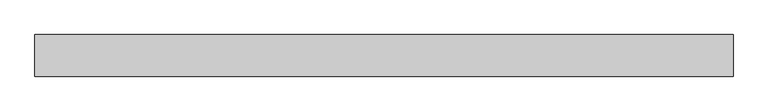
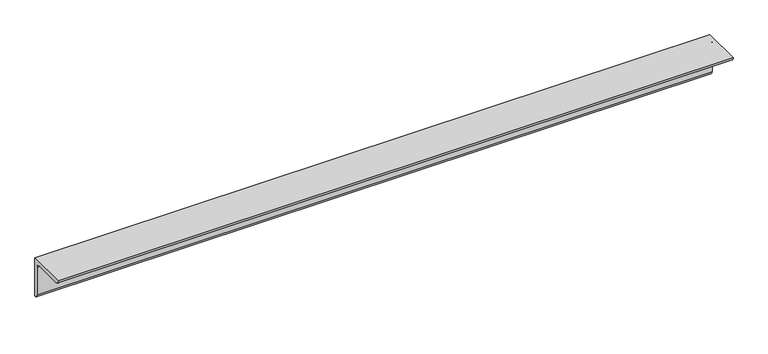
"""IFC4 building model written with IfcOpenShell, lengths in millimetres: member geometry, 0912_Steel Framing_L-KSD3502 : H_SB_AR_S03_L-130x130x12_HBR3."""

from ifc_helpers import new_model, si_unit, point, frame, frame_2d, origin, place, context, project, spatial, polyline, circle_curve, trimmed, segment, composite_curve, outline, extrude, source, transform, mapped, element, save


def member_70962aff(model_context):
    return source(origin(), model_context, "Body", "SweptSolid", [
        extrude(outline(composite_curve([segment(polyline([(36.4, 36.4), (36.4, -93.6)]), True, "CONTINUOUS"), segment(trimmed(circle_curve(frame_2d((36.4, -81.6)), 12.0), [point((36.4, -93.6))], [point((24.4, -81.6))], False, "CARTESIAN"), True, "CONTINUOUS"), segment(polyline([(24.4, -81.6), (24.4, 12.4)]), True, "CONTINUOUS"), segment(trimmed(circle_curve(frame_2d((12.4, 12.4)), 12.0), [point((24.4, 12.4))], [point((12.4, 24.4))], True, "CARTESIAN"), True, "CONTINUOUS"), segment(polyline([(12.4, 24.4), (-81.6, 24.4)]), True, "CONTINUOUS"), segment(trimmed(circle_curve(frame_2d((-81.6, 36.4)), 12.0), [point((-81.6, 24.4))], [point((-93.6, 36.4))], False, "CARTESIAN"), True, "CONTINUOUS"), segment(polyline([(-93.6, 36.4), (36.4, 36.4)]), True, "CONTINUOUS")], self_intersect=False)), frame((-995.2380761, 0.0, 0.0), z_axis=(1.0, 0.0, 0.0), x_axis=(0.0, 1.0, 0.0)), (0.0, 0.0, 1.0), 2181.7834935),
    ])


if __name__ == "__main__":
    model = new_model("IFC4")
    model_context = context("Model", 3, world=origin())
    ifc_project = project(units=[si_unit("LENGTHUNIT", "METRE", prefix="MILLI")], contexts=[model_context])
    site = spatial("IfcSite", under=ifc_project)
    building = spatial("IfcBuilding", under=site)
    placement = place(None, origin())
    member_shape = member_70962aff(model_context)
    element("IfcMember", 1, ObjectType="0912_Steel Framing_L-KSD3502 : H_SB_AR_S03_L-130x130x12_HBR3", at=placement, inside=building, context=model_context, shape_type="MappedRepresentation", body=[
        mapped(member_shape, transform((0.0, 0.0, 0.0), x_axis=(1.0, 0.0, 0.0), y_axis=(0.0, 1.0, 0.0), z_axis=(0.0, 0.0, 1.0))),
    ])
    save(model, "model.ifc")

# Revit data of these elements
# Type "0912_Steel Framing_L-KSD3502 : H_SB_AR_S03_L-130x130x12_HBR3"
#   k = 25 mm
#   Perimeter = 0.52 m²/m
#   Nominal Weight = 23.40 kgf/m
#   Length [instance default] = 1000 mm
#   b = 130 mm
#   d = 130 mm
#   t = 12 mm
#   x = 36.4 mm
#   y = 36.4 mm
#   A = 2976.00 m²
#   Structural Material [instance default] = Steel, 45-345
# Element 1 (IfcMember, "0912_Steel Framing_L-KSD3502 : H_SB_AR_S03_L-130x130x12_HBR3")
#   Structural Material = Steel ASTM A36
#   Materials on its faces: "Steel ASTM A36"
# Materials
#   "Steel, 45-345": class "Metal", colour RGB 189 187 185, transparency 0, Description = "Steel 345 MPa", Cost = 0
#   "Steel ASTM A36": class "Metal", colour RGB 199 199 199, transparency 0, Description = "Structural steel, ASTM A36 Grade B, mill finish", Cost = 0
